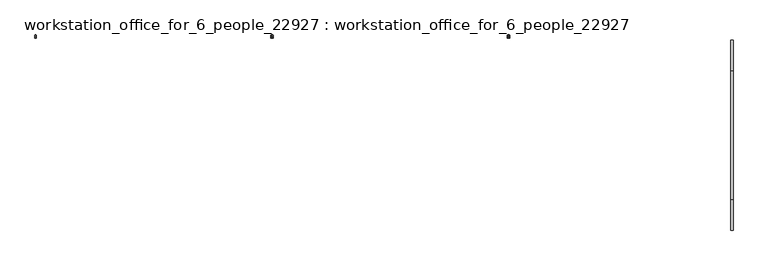
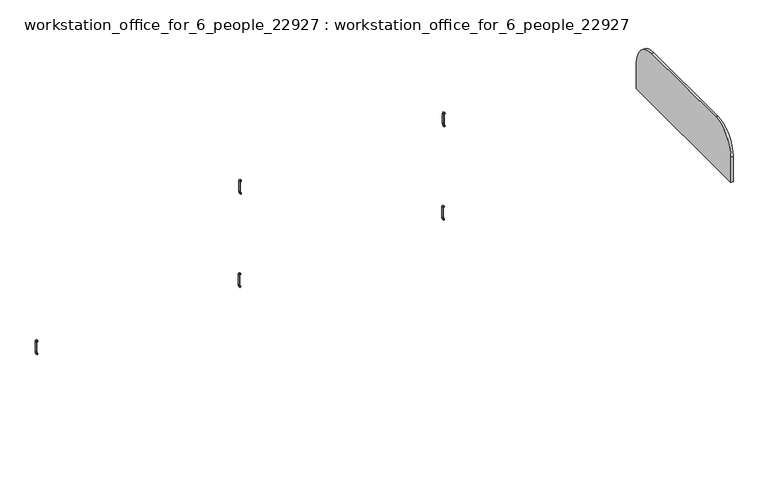
"""IFC4 building model written with IfcOpenShell, lengths in millimetres: proxy geometry, workstation_office_for_6_people_22927 : workstation_office_for_6_people_22927."""

from ifc_helpers import new_model, si_unit, point, frame, frame_2d, origin, place, context, project, spatial, polyline, circle_curve, ellipse_curve, trimmed, segment, composite_curve, outline, extrude, source, transform, mapped, element, save
from ifc_brep_helpers import plane_surface, cylinder_surface, revolved_surface, advanced_brep


def workstation_office_for_6_people_22927_workstation_office_for_d460ba9c(model_context):
    return source(origin(), model_context, "Body", "SolidModel", [
        advanced_brep(
        [(-850.0, 629.8015658, 350.0), (-850.0, 629.8015658, 360.0), (-850.0, 635.0, 360.0), (-850.0, 635.0, 350.0), (-850.0, 640.0, 345.0), (-850.0, 650.0, 345.0), (-850.0, 650.0, 265.0), (-850.0, 640.0, 265.0), (-850.0, 635.0, 260.0), (-850.0, 635.0, 250.0), (-850.0, 629.8015658, 260.0), (-850.0, 629.8015658, 250.0)],
        [
            (0, 1, circle_curve(frame((-850.0, 629.8015658, 355.0), z_axis=(0.0, -1.0, 0.0), x_axis=(0.0, 0.0, 1.0)), 5.0)),
            (1, 0, circle_curve(frame((-850.0, 629.8015658, 355.0), z_axis=(0.0, -1.0, 0.0), x_axis=(0.0, 0.0, 1.0)), 5.0)),
            (1, 2),
            (2, 3, circle_curve(frame((-850.0, 635.0, 355.0), z_axis=(0.0, -1.0, 0.0), x_axis=(0.0, 0.0, 1.0)), 5.0)),
            (3, 0),
            (3, 2, circle_curve(frame((-850.0, 635.0, 355.0), z_axis=(0.0, -1.0, 0.0), x_axis=(0.0, 0.0, 1.0)), 5.0)),
            (4, 3, circle_curve(frame((-850.0, 635.0, 345.0), z_axis=(1.0, 0.0, 0.0), x_axis=(0.0, 0.0, 1.0)), 5.0)),
            (2, 5, circle_curve(frame((-850.0, 635.0, 345.0), z_axis=(-1.0, 0.0, 0.0), x_axis=(0.0, 0.0, 1.0)), 15.0)),
            (5, 4, circle_curve(frame((-850.0, 645.0, 345.0), z_axis=(0.0, 0.0, 1.0), x_axis=(0.0, 1.0, 0.0)), 5.0)),
            (4, 5, circle_curve(frame((-850.0, 645.0, 345.0), z_axis=(0.0, 0.0, 1.0), x_axis=(0.0, 1.0, 0.0)), 5.0)),
            (5, 6),
            (6, 7, circle_curve(frame((-850.0, 645.0, 265.0), z_axis=(0.0, 0.0, 1.0), x_axis=(0.0, 1.0, 0.0)), 5.0)),
            (7, 4),
            (7, 6, circle_curve(frame((-850.0, 645.0, 265.0), z_axis=(0.0, 0.0, 1.0), x_axis=(0.0, 1.0, 0.0)), 5.0)),
            (8, 7, circle_curve(frame((-850.0, 635.0, 265.0), z_axis=(1.0, 0.0, 0.0), x_axis=(0.0, 1.0, 0.0)), 5.0)),
            (6, 9, circle_curve(frame((-850.0, 635.0, 265.0), z_axis=(-1.0, 0.0, 0.0), x_axis=(0.0, 1.0, 0.0)), 15.0)),
            (9, 8, circle_curve(frame((-850.0, 635.0, 255.0), z_axis=(0.0, 1.0, 0.0), x_axis=(0.0, 0.0, -1.0)), 5.0)),
            (8, 9, circle_curve(frame((-850.0, 635.0, 255.0), z_axis=(0.0, 1.0, 0.0), x_axis=(0.0, 0.0, -1.0)), 5.0)),
            (10, 11, circle_curve(frame((-850.0, 629.8015658, 255.0), z_axis=(0.0, -1.0, 0.0), x_axis=(0.0, 0.0, -1.0)), 5.0)),
            (11, 10, circle_curve(frame((-850.0, 629.8015658, 255.0), z_axis=(0.0, -1.0, 0.0), x_axis=(0.0, 0.0, -1.0)), 5.0)),
            (9, 11),
            (10, 8),
        ],
        [
            plane_surface(frame((0.0, 629.8015658, 355.0), z_axis=(0.0, -1.0, 0.0), x_axis=(1.0, 0.0, 0.0))),
            cylinder_surface(frame((-850.0, 629.8015658, 355.0), z_axis=(0.0, -1.0, 0.0), x_axis=(0.0, 0.0, 1.0)), 5.0),
            revolved_surface(trimmed(ellipse_curve(frame((-850.0, 635.0, 355.0), z_axis=(0.0, -1.0, 0.0), x_axis=(0.0, 0.0, 1.0)), 5.0, 5.0), [point((-850.0, 635.0, 360.0))], [point((-850.0, 635.0, 350.0))], True, "CARTESIAN"), (0.0, 635.0, 345.0), (-1.0, 0.0, 0.0)),
            revolved_surface(trimmed(ellipse_curve(frame((-850.0, 635.0, 355.0), z_axis=(0.0, -1.0, 0.0), x_axis=(0.0, 0.0, 1.0)), 5.0, 5.0), [point((-850.0, 635.0, 350.0))], [point((-850.0, 635.0, 360.0))], True, "CARTESIAN"), (0.0, 635.0, 345.0), (-1.0, 0.0, 0.0)),
            cylinder_surface(frame((-850.0, 645.0, 345.0), z_axis=(0.0, 0.0, 1.0), x_axis=(0.0, 1.0, 0.0)), 5.0),
            revolved_surface(trimmed(ellipse_curve(frame((-850.0, 645.0, 265.0), z_axis=(0.0, 0.0, 1.0), x_axis=(0.0, 1.0, 0.0)), 5.0, 5.0), [point((-850.0, 650.0, 265.0))], [point((-850.0, 640.0, 265.0))], True, "CARTESIAN"), (0.0, 635.0, 265.0), (-1.0, 0.0, 0.0)),
            revolved_surface(trimmed(ellipse_curve(frame((-850.0, 645.0, 265.0), z_axis=(0.0, 0.0, 1.0), x_axis=(0.0, 1.0, 0.0)), 5.0, 5.0), [point((-850.0, 640.0, 265.0))], [point((-850.0, 650.0, 265.0))], True, "CARTESIAN"), (0.0, 635.0, 265.0), (-1.0, 0.0, 0.0)),
            plane_surface(frame((0.0, 629.8015658, 255.0), z_axis=(0.0, -1.0, 0.0), x_axis=(1.0, 0.0, 0.0))),
            cylinder_surface(frame((-850.0, 635.0, 255.0), z_axis=(0.0, 1.0, 0.0), x_axis=(0.0, 0.0, -1.0)), 5.0),
        ],
        [
            (0, [[1, 2]]),
            (1, [[-2, 3, 4, 5]]),
            (1, [[-1, -5, 6, -3]]),
            (2, [[7, -4, 8, 9]]),
            (3, [[-8, -6, -7, 10]]),
            (4, [[-9, 11, 12, 13]]),
            (4, [[-10, -13, 14, -11]]),
            (5, [[15, -12, 16, 17]]),
            (6, [[-16, -14, -15, 18]]),
            (7, [[19, 20]]),
            (8, [[-17, 21, -19, 22]]),
            (8, [[-18, -22, -20, -21]]),
        ],
    ),
        advanced_brep(
        [(680.0, 629.8015658, 1090.0), (680.0, 629.8015658, 1100.0), (680.0, 635.0, 1100.0), (680.0, 635.0, 1090.0), (680.0, 640.0, 1085.0), (680.0, 650.0, 1085.0), (680.0, 650.0, 1005.0), (680.0, 640.0, 1005.0), (680.0, 635.0, 1000.0), (680.0, 635.0, 990.0), (680.0, 629.8015658, 1000.0), (680.0, 629.8015658, 990.0)],
        [
            (0, 1, circle_curve(frame((680.0, 629.8015658, 1095.0), z_axis=(0.0, -1.0, 0.0), x_axis=(0.0, 0.0, 1.0)), 5.0)),
            (1, 0, circle_curve(frame((680.0, 629.8015658, 1095.0), z_axis=(0.0, -1.0, 0.0), x_axis=(0.0, 0.0, 1.0)), 5.0)),
            (1, 2),
            (2, 3, circle_curve(frame((680.0, 635.0, 1095.0), z_axis=(0.0, -1.0, 0.0), x_axis=(0.0, 0.0, 1.0)), 5.0)),
            (3, 0),
            (3, 2, circle_curve(frame((680.0, 635.0, 1095.0), z_axis=(0.0, -1.0, 0.0), x_axis=(0.0, 0.0, 1.0)), 5.0)),
            (4, 3, circle_curve(frame((680.0, 635.0, 1085.0), z_axis=(1.0, 0.0, 0.0), x_axis=(0.0, 0.0, 1.0)), 5.0)),
            (2, 5, circle_curve(frame((680.0, 635.0, 1085.0), z_axis=(-1.0, 0.0, 0.0), x_axis=(0.0, 0.0, 1.0)), 15.0)),
            (5, 4, circle_curve(frame((680.0, 645.0, 1085.0), z_axis=(0.0, 0.0, 1.0), x_axis=(0.0, 1.0, 0.0)), 5.0)),
            (4, 5, circle_curve(frame((680.0, 645.0, 1085.0), z_axis=(0.0, 0.0, 1.0), x_axis=(0.0, 1.0, 0.0)), 5.0)),
            (5, 6),
            (6, 7, circle_curve(frame((680.0, 645.0, 1005.0), z_axis=(0.0, 0.0, 1.0), x_axis=(0.0, 1.0, 0.0)), 5.0)),
            (7, 4),
            (7, 6, circle_curve(frame((680.0, 645.0, 1005.0), z_axis=(0.0, 0.0, 1.0), x_axis=(0.0, 1.0, 0.0)), 5.0)),
            (8, 7, circle_curve(frame((680.0, 635.0, 1005.0), z_axis=(1.0, 0.0, 0.0), x_axis=(0.0, 1.0, 0.0)), 5.0)),
            (6, 9, circle_curve(frame((680.0, 635.0, 1005.0), z_axis=(-1.0, 0.0, 0.0), x_axis=(0.0, 1.0, 0.0)), 15.0)),
            (9, 8, circle_curve(frame((680.0, 635.0, 995.0), z_axis=(0.0, 1.0, 0.0), x_axis=(0.0, 0.0, -1.0)), 5.0)),
            (8, 9, circle_curve(frame((680.0, 635.0, 995.0), z_axis=(0.0, 1.0, 0.0), x_axis=(0.0, 0.0, -1.0)), 5.0)),
            (10, 11, circle_curve(frame((680.0, 629.8015658, 995.0), z_axis=(0.0, -1.0, 0.0), x_axis=(0.0, 0.0, -1.0)), 5.0)),
            (11, 10, circle_curve(frame((680.0, 629.8015658, 995.0), z_axis=(0.0, -1.0, 0.0), x_axis=(0.0, 0.0, -1.0)), 5.0)),
            (9, 11),
            (10, 8),
        ],
        [
            plane_surface(frame((1530.0, 629.8015658, 1095.0), z_axis=(0.0, -1.0, 0.0), x_axis=(1.0, 0.0, 0.0))),
            cylinder_surface(frame((680.0, 629.8015658, 1095.0), z_axis=(0.0, -1.0, 0.0), x_axis=(0.0, 0.0, 1.0)), 5.0),
            revolved_surface(trimmed(ellipse_curve(frame((680.0, 635.0, 1095.0), z_axis=(0.0, -1.0, 0.0), x_axis=(0.0, 0.0, 1.0)), 5.0, 5.0), [point((680.0, 635.0, 1100.0))], [point((680.0, 635.0, 1090.0))], True, "CARTESIAN"), (1530.0, 635.0, 1085.0), (-1.0, 0.0, 0.0)),
            revolved_surface(trimmed(ellipse_curve(frame((680.0, 635.0, 1095.0), z_axis=(0.0, -1.0, 0.0), x_axis=(0.0, 0.0, 1.0)), 5.0, 5.0), [point((680.0, 635.0, 1090.0))], [point((680.0, 635.0, 1100.0))], True, "CARTESIAN"), (1530.0, 635.0, 1085.0), (-1.0, 0.0, 0.0)),
            cylinder_surface(frame((680.0, 645.0, 1085.0), z_axis=(0.0, 0.0, 1.0), x_axis=(0.0, 1.0, 0.0)), 5.0),
            revolved_surface(trimmed(ellipse_curve(frame((680.0, 645.0, 1005.0), z_axis=(0.0, 0.0, 1.0), x_axis=(0.0, 1.0, 0.0)), 5.0, 5.0), [point((680.0, 650.0, 1005.0))], [point((680.0, 640.0, 1005.0))], True, "CARTESIAN"), (1530.0, 635.0, 1005.0), (-1.0, 0.0, 0.0)),
            revolved_surface(trimmed(ellipse_curve(frame((680.0, 645.0, 1005.0), z_axis=(0.0, 0.0, 1.0), x_axis=(0.0, 1.0, 0.0)), 5.0, 5.0), [point((680.0, 640.0, 1005.0))], [point((680.0, 650.0, 1005.0))], True, "CARTESIAN"), (1530.0, 635.0, 1005.0), (-1.0, 0.0, 0.0)),
            plane_surface(frame((1530.0, 629.8015658, 995.0), z_axis=(0.0, -1.0, 0.0), x_axis=(1.0, 0.0, 0.0))),
            cylinder_surface(frame((680.0, 635.0, 995.0), z_axis=(0.0, 1.0, 0.0), x_axis=(0.0, 0.0, -1.0)), 5.0),
        ],
        [
            (0, [[1, 2]]),
            (1, [[-2, 3, 4, 5]]),
            (1, [[-1, -5, 6, -3]]),
            (2, [[7, -4, 8, 9]]),
            (3, [[-8, -6, -7, 10]]),
            (4, [[-9, 11, 12, 13]]),
            (4, [[-10, -13, 14, -11]]),
            (5, [[15, -12, 16, 17]]),
            (6, [[-16, -14, -15, 18]]),
            (7, [[19, 20]]),
            (8, [[-17, 21, -19, 22]]),
            (8, [[-18, -22, -20, -21]]),
        ],
    ),
        advanced_brep(
        [(675.0, 629.8015658, 350.0), (675.0, 629.8015658, 360.0), (675.0, 635.0, 360.0), (675.0, 635.0, 350.0), (675.0, 640.0, 345.0), (675.0, 650.0, 345.0), (675.0, 650.0, 265.0), (675.0, 640.0, 265.0), (675.0, 635.0, 260.0), (675.0, 635.0, 250.0), (675.0, 629.8015658, 260.0), (675.0, 629.8015658, 250.0)],
        [
            (0, 1, circle_curve(frame((675.0, 629.8015658, 355.0), z_axis=(0.0, -1.0, 0.0), x_axis=(0.0, 0.0, 1.0)), 5.0)),
            (1, 0, circle_curve(frame((675.0, 629.8015658, 355.0), z_axis=(0.0, -1.0, 0.0), x_axis=(0.0, 0.0, 1.0)), 5.0)),
            (1, 2),
            (2, 3, circle_curve(frame((675.0, 635.0, 355.0), z_axis=(0.0, -1.0, 0.0), x_axis=(0.0, 0.0, 1.0)), 5.0)),
            (3, 0),
            (3, 2, circle_curve(frame((675.0, 635.0, 355.0), z_axis=(0.0, -1.0, 0.0), x_axis=(0.0, 0.0, 1.0)), 5.0)),
            (4, 3, circle_curve(frame((675.0, 635.0, 345.0), z_axis=(1.0, 0.0, 0.0), x_axis=(0.0, 0.0, 1.0)), 5.0)),
            (2, 5, circle_curve(frame((675.0, 635.0, 345.0), z_axis=(-1.0, 0.0, 0.0), x_axis=(0.0, 0.0, 1.0)), 15.0)),
            (5, 4, circle_curve(frame((675.0, 645.0, 345.0), z_axis=(0.0, 0.0, 1.0), x_axis=(0.0, 1.0, 0.0)), 5.0)),
            (4, 5, circle_curve(frame((675.0, 645.0, 345.0), z_axis=(0.0, 0.0, 1.0), x_axis=(0.0, 1.0, 0.0)), 5.0)),
            (5, 6),
            (6, 7, circle_curve(frame((675.0, 645.0, 265.0), z_axis=(0.0, 0.0, 1.0), x_axis=(0.0, 1.0, 0.0)), 5.0)),
            (7, 4),
            (7, 6, circle_curve(frame((675.0, 645.0, 265.0), z_axis=(0.0, 0.0, 1.0), x_axis=(0.0, 1.0, 0.0)), 5.0)),
            (8, 7, circle_curve(frame((675.0, 635.0, 265.0), z_axis=(1.0, 0.0, 0.0), x_axis=(0.0, 1.0, 0.0)), 5.0)),
            (6, 9, circle_curve(frame((675.0, 635.0, 265.0), z_axis=(-1.0, 0.0, 0.0), x_axis=(0.0, 1.0, 0.0)), 15.0)),
            (9, 8, circle_curve(frame((675.0, 635.0, 255.0), z_axis=(0.0, 1.0, 0.0), x_axis=(0.0, 0.0, -1.0)), 5.0)),
            (8, 9, circle_curve(frame((675.0, 635.0, 255.0), z_axis=(0.0, 1.0, 0.0), x_axis=(0.0, 0.0, -1.0)), 5.0)),
            (10, 11, circle_curve(frame((675.0, 629.8015658, 255.0), z_axis=(0.0, -1.0, 0.0), x_axis=(0.0, 0.0, -1.0)), 5.0)),
            (11, 10, circle_curve(frame((675.0, 629.8015658, 255.0), z_axis=(0.0, -1.0, 0.0), x_axis=(0.0, 0.0, -1.0)), 5.0)),
            (9, 11),
            (10, 8),
        ],
        [
            plane_surface(frame((675.0, 629.8015658, 355.0), z_axis=(0.0, -1.0, 0.0), x_axis=(1.0, 0.0, 0.0))),
            cylinder_surface(frame((675.0, 629.8015658, 355.0), z_axis=(0.0, -1.0, 0.0), x_axis=(0.0, 0.0, 1.0)), 5.0),
            revolved_surface(trimmed(ellipse_curve(frame((675.0, 635.0, 355.0), z_axis=(0.0, -1.0, 0.0), x_axis=(0.0, 0.0, 1.0)), 5.0, 5.0), [point((675.0, 635.0, 360.0))], [point((675.0, 635.0, 350.0))], True, "CARTESIAN"), (675.0, 635.0, 345.0), (-1.0, 0.0, 0.0)),
            revolved_surface(trimmed(ellipse_curve(frame((675.0, 635.0, 355.0), z_axis=(0.0, -1.0, 0.0), x_axis=(0.0, 0.0, 1.0)), 5.0, 5.0), [point((675.0, 635.0, 350.0))], [point((675.0, 635.0, 360.0))], True, "CARTESIAN"), (675.0, 635.0, 345.0), (-1.0, 0.0, 0.0)),
            cylinder_surface(frame((675.0, 645.0, 345.0), z_axis=(0.0, 0.0, 1.0), x_axis=(0.0, 1.0, 0.0)), 5.0),
            revolved_surface(trimmed(ellipse_curve(frame((675.0, 645.0, 265.0), z_axis=(0.0, 0.0, 1.0), x_axis=(0.0, 1.0, 0.0)), 5.0, 5.0), [point((675.0, 650.0, 265.0))], [point((675.0, 640.0, 265.0))], True, "CARTESIAN"), (675.0, 635.0, 265.0), (-1.0, 0.0, 0.0)),
            revolved_surface(trimmed(ellipse_curve(frame((675.0, 645.0, 265.0), z_axis=(0.0, 0.0, 1.0), x_axis=(0.0, 1.0, 0.0)), 5.0, 5.0), [point((675.0, 640.0, 265.0))], [point((675.0, 650.0, 265.0))], True, "CARTESIAN"), (675.0, 635.0, 265.0), (-1.0, 0.0, 0.0)),
            plane_surface(frame((675.0, 629.8015658, 255.0), z_axis=(0.0, -1.0, 0.0), x_axis=(1.0, 0.0, 0.0))),
            cylinder_surface(frame((675.0, 635.0, 255.0), z_axis=(0.0, 1.0, 0.0), x_axis=(0.0, 0.0, -1.0)), 5.0),
        ],
        [
            (0, [[1, 2]]),
            (1, [[-2, 3, 4, 5]]),
            (1, [[-1, -5, 6, -3]]),
            (2, [[7, -4, 8, 9]]),
            (3, [[-8, -6, -7, 10]]),
            (4, [[-9, 11, 12, 13]]),
            (4, [[-10, -13, 14, -11]]),
            (5, [[15, -12, 16, 17]]),
            (6, [[-16, -14, -15, 18]]),
            (7, [[19, 20]]),
            (8, [[-17, 21, -19, 22]]),
            (8, [[-18, -22, -20, -21]]),
        ],
    ),
        advanced_brep(
        [(2210.0, 629.8015658, 1090.0), (2210.0, 629.8015658, 1100.0), (2210.0, 635.0, 1100.0), (2210.0, 635.0, 1090.0), (2210.0, 640.0, 1085.0), (2210.0, 650.0, 1085.0), (2210.0, 650.0, 1005.0), (2210.0, 640.0, 1005.0), (2210.0, 635.0, 1000.0), (2210.0, 635.0, 990.0), (2210.0, 629.8015658, 1000.0), (2210.0, 629.8015658, 990.0)],
        [
            (0, 1, circle_curve(frame((2210.0, 629.8015658, 1095.0), z_axis=(0.0, -1.0, 0.0), x_axis=(0.0, 0.0, 1.0)), 5.0)),
            (1, 0, circle_curve(frame((2210.0, 629.8015658, 1095.0), z_axis=(0.0, -1.0, 0.0), x_axis=(0.0, 0.0, 1.0)), 5.0)),
            (1, 2),
            (2, 3, circle_curve(frame((2210.0, 635.0, 1095.0), z_axis=(0.0, -1.0, 0.0), x_axis=(0.0, 0.0, 1.0)), 5.0)),
            (3, 0),
            (3, 2, circle_curve(frame((2210.0, 635.0, 1095.0), z_axis=(0.0, -1.0, 0.0), x_axis=(0.0, 0.0, 1.0)), 5.0)),
            (4, 3, circle_curve(frame((2210.0, 635.0, 1085.0), z_axis=(1.0, 0.0, 0.0), x_axis=(0.0, 0.0, 1.0)), 5.0)),
            (2, 5, circle_curve(frame((2210.0, 635.0, 1085.0), z_axis=(-1.0, 0.0, 0.0), x_axis=(0.0, 0.0, 1.0)), 15.0)),
            (5, 4, circle_curve(frame((2210.0, 645.0, 1085.0), z_axis=(0.0, 0.0, 1.0), x_axis=(0.0, 1.0, 0.0)), 5.0)),
            (4, 5, circle_curve(frame((2210.0, 645.0, 1085.0), z_axis=(0.0, 0.0, 1.0), x_axis=(0.0, 1.0, 0.0)), 5.0)),
            (5, 6),
            (6, 7, circle_curve(frame((2210.0, 645.0, 1005.0), z_axis=(0.0, 0.0, 1.0), x_axis=(0.0, 1.0, 0.0)), 5.0)),
            (7, 4),
            (7, 6, circle_curve(frame((2210.0, 645.0, 1005.0), z_axis=(0.0, 0.0, 1.0), x_axis=(0.0, 1.0, 0.0)), 5.0)),
            (8, 7, circle_curve(frame((2210.0, 635.0, 1005.0), z_axis=(1.0, 0.0, 0.0), x_axis=(0.0, 1.0, 0.0)), 5.0)),
            (6, 9, circle_curve(frame((2210.0, 635.0, 1005.0), z_axis=(-1.0, 0.0, 0.0), x_axis=(0.0, 1.0, 0.0)), 15.0)),
            (9, 8, circle_curve(frame((2210.0, 635.0, 995.0), z_axis=(0.0, 1.0, 0.0), x_axis=(0.0, 0.0, -1.0)), 5.0)),
            (8, 9, circle_curve(frame((2210.0, 635.0, 995.0), z_axis=(0.0, 1.0, 0.0), x_axis=(0.0, 0.0, -1.0)), 5.0)),
            (10, 11, circle_curve(frame((2210.0, 629.8015658, 995.0), z_axis=(0.0, -1.0, 0.0), x_axis=(0.0, 0.0, -1.0)), 5.0)),
            (11, 10, circle_curve(frame((2210.0, 629.8015658, 995.0), z_axis=(0.0, -1.0, 0.0), x_axis=(0.0, 0.0, -1.0)), 5.0)),
            (9, 11),
            (10, 8),
        ],
        [
            plane_surface(frame((3060.0, 629.8015658, 1095.0), z_axis=(0.0, -1.0, 0.0), x_axis=(1.0, 0.0, 0.0))),
            cylinder_surface(frame((2210.0, 629.8015658, 1095.0), z_axis=(0.0, -1.0, 0.0), x_axis=(0.0, 0.0, 1.0)), 5.0),
            revolved_surface(trimmed(ellipse_curve(frame((2210.0, 635.0, 1095.0), z_axis=(0.0, -1.0, 0.0), x_axis=(0.0, 0.0, 1.0)), 5.0, 5.0), [point((2210.0, 635.0, 1100.0))], [point((2210.0, 635.0, 1090.0))], True, "CARTESIAN"), (3060.0, 635.0, 1085.0), (-1.0, 0.0, 0.0)),
            revolved_surface(trimmed(ellipse_curve(frame((2210.0, 635.0, 1095.0), z_axis=(0.0, -1.0, 0.0), x_axis=(0.0, 0.0, 1.0)), 5.0, 5.0), [point((2210.0, 635.0, 1090.0))], [point((2210.0, 635.0, 1100.0))], True, "CARTESIAN"), (3060.0, 635.0, 1085.0), (-1.0, 0.0, 0.0)),
            cylinder_surface(frame((2210.0, 645.0, 1085.0), z_axis=(0.0, 0.0, 1.0), x_axis=(0.0, 1.0, 0.0)), 5.0),
            revolved_surface(trimmed(ellipse_curve(frame((2210.0, 645.0, 1005.0), z_axis=(0.0, 0.0, 1.0), x_axis=(0.0, 1.0, 0.0)), 5.0, 5.0), [point((2210.0, 650.0, 1005.0))], [point((2210.0, 640.0, 1005.0))], True, "CARTESIAN"), (3060.0, 635.0, 1005.0), (-1.0, 0.0, 0.0)),
            revolved_surface(trimmed(ellipse_curve(frame((2210.0, 645.0, 1005.0), z_axis=(0.0, 0.0, 1.0), x_axis=(0.0, 1.0, 0.0)), 5.0, 5.0), [point((2210.0, 640.0, 1005.0))], [point((2210.0, 650.0, 1005.0))], True, "CARTESIAN"), (3060.0, 635.0, 1005.0), (-1.0, 0.0, 0.0)),
            plane_surface(frame((3060.0, 629.8015658, 995.0), z_axis=(0.0, -1.0, 0.0), x_axis=(1.0, 0.0, 0.0))),
            cylinder_surface(frame((2210.0, 635.0, 995.0), z_axis=(0.0, 1.0, 0.0), x_axis=(0.0, 0.0, -1.0)), 5.0),
        ],
        [
            (0, [[1, 2]]),
            (1, [[-2, 3, 4, 5]]),
            (1, [[-1, -5, 6, -3]]),
            (2, [[7, -4, 8, 9]]),
            (3, [[-8, -6, -7, 10]]),
            (4, [[-9, 11, 12, 13]]),
            (4, [[-10, -13, 14, -11]]),
            (5, [[15, -12, 16, 17]]),
            (6, [[-16, -14, -15, 18]]),
            (7, [[19, 20]]),
            (8, [[-17, 21, -19, 22]]),
            (8, [[-18, -22, -20, -21]]),
        ],
    ),
        advanced_brep(
        [(2205.0, 629.8015658, 350.0), (2205.0, 629.8015658, 360.0), (2205.0, 635.0, 360.0), (2205.0, 635.0, 350.0), (2205.0, 640.0, 345.0), (2205.0, 650.0, 345.0), (2205.0, 650.0, 265.0), (2205.0, 640.0, 265.0), (2205.0, 635.0, 260.0), (2205.0, 635.0, 250.0), (2205.0, 629.8015658, 260.0), (2205.0, 629.8015658, 250.0)],
        [
            (0, 1, circle_curve(frame((2205.0, 629.8015658, 355.0), z_axis=(0.0, -1.0, 0.0), x_axis=(0.0, 0.0, 1.0)), 5.0)),
            (1, 0, circle_curve(frame((2205.0, 629.8015658, 355.0), z_axis=(0.0, -1.0, 0.0), x_axis=(0.0, 0.0, 1.0)), 5.0)),
            (1, 2),
            (2, 3, circle_curve(frame((2205.0, 635.0, 355.0), z_axis=(0.0, -1.0, 0.0), x_axis=(0.0, 0.0, 1.0)), 5.0)),
            (3, 0),
            (3, 2, circle_curve(frame((2205.0, 635.0, 355.0), z_axis=(0.0, -1.0, 0.0), x_axis=(0.0, 0.0, 1.0)), 5.0)),
            (4, 3, circle_curve(frame((2205.0, 635.0, 345.0), z_axis=(1.0, 0.0, 0.0), x_axis=(0.0, 0.0, 1.0)), 5.0)),
            (2, 5, circle_curve(frame((2205.0, 635.0, 345.0), z_axis=(-1.0, 0.0, 0.0), x_axis=(0.0, 0.0, 1.0)), 15.0)),
            (5, 4, circle_curve(frame((2205.0, 645.0, 345.0), z_axis=(0.0, 0.0, 1.0), x_axis=(0.0, 1.0, 0.0)), 5.0)),
            (4, 5, circle_curve(frame((2205.0, 645.0, 345.0), z_axis=(0.0, 0.0, 1.0), x_axis=(0.0, 1.0, 0.0)), 5.0)),
            (5, 6),
            (6, 7, circle_curve(frame((2205.0, 645.0, 265.0), z_axis=(0.0, 0.0, 1.0), x_axis=(0.0, 1.0, 0.0)), 5.0)),
            (7, 4),
            (7, 6, circle_curve(frame((2205.0, 645.0, 265.0), z_axis=(0.0, 0.0, 1.0), x_axis=(0.0, 1.0, 0.0)), 5.0)),
            (8, 7, circle_curve(frame((2205.0, 635.0, 265.0), z_axis=(1.0, 0.0, 0.0), x_axis=(0.0, 1.0, 0.0)), 5.0)),
            (6, 9, circle_curve(frame((2205.0, 635.0, 265.0), z_axis=(-1.0, 0.0, 0.0), x_axis=(0.0, 1.0, 0.0)), 15.0)),
            (9, 8, circle_curve(frame((2205.0, 635.0, 255.0), z_axis=(0.0, 1.0, 0.0), x_axis=(0.0, 0.0, -1.0)), 5.0)),
            (8, 9, circle_curve(frame((2205.0, 635.0, 255.0), z_axis=(0.0, 1.0, 0.0), x_axis=(0.0, 0.0, -1.0)), 5.0)),
            (10, 11, circle_curve(frame((2205.0, 629.8015658, 255.0), z_axis=(0.0, -1.0, 0.0), x_axis=(0.0, 0.0, -1.0)), 5.0)),
            (11, 10, circle_curve(frame((2205.0, 629.8015658, 255.0), z_axis=(0.0, -1.0, 0.0), x_axis=(0.0, 0.0, -1.0)), 5.0)),
            (9, 11),
            (10, 8),
        ],
        [
            plane_surface(frame((2205.0, 629.8015658, 355.0), z_axis=(0.0, -1.0, 0.0), x_axis=(1.0, 0.0, 0.0))),
            cylinder_surface(frame((2205.0, 629.8015658, 355.0), z_axis=(0.0, -1.0, 0.0), x_axis=(0.0, 0.0, 1.0)), 5.0),
            revolved_surface(trimmed(ellipse_curve(frame((2205.0, 635.0, 355.0), z_axis=(0.0, -1.0, 0.0), x_axis=(0.0, 0.0, 1.0)), 5.0, 5.0), [point((2205.0, 635.0, 360.0))], [point((2205.0, 635.0, 350.0))], True, "CARTESIAN"), (2205.0, 635.0, 345.0), (-1.0, 0.0, 0.0)),
            revolved_surface(trimmed(ellipse_curve(frame((2205.0, 635.0, 355.0), z_axis=(0.0, -1.0, 0.0), x_axis=(0.0, 0.0, 1.0)), 5.0, 5.0), [point((2205.0, 635.0, 350.0))], [point((2205.0, 635.0, 360.0))], True, "CARTESIAN"), (2205.0, 635.0, 345.0), (-1.0, 0.0, 0.0)),
            cylinder_surface(frame((2205.0, 645.0, 345.0), z_axis=(0.0, 0.0, 1.0), x_axis=(0.0, 1.0, 0.0)), 5.0),
            revolved_surface(trimmed(ellipse_curve(frame((2205.0, 645.0, 265.0), z_axis=(0.0, 0.0, 1.0), x_axis=(0.0, 1.0, 0.0)), 5.0, 5.0), [point((2205.0, 650.0, 265.0))], [point((2205.0, 640.0, 265.0))], True, "CARTESIAN"), (2205.0, 635.0, 265.0), (-1.0, 0.0, 0.0)),
            revolved_surface(trimmed(ellipse_curve(frame((2205.0, 645.0, 265.0), z_axis=(0.0, 0.0, 1.0), x_axis=(0.0, 1.0, 0.0)), 5.0, 5.0), [point((2205.0, 640.0, 265.0))], [point((2205.0, 650.0, 265.0))], True, "CARTESIAN"), (2205.0, 635.0, 265.0), (-1.0, 0.0, 0.0)),
            plane_surface(frame((2205.0, 629.8015658, 255.0), z_axis=(0.0, -1.0, 0.0), x_axis=(1.0, 0.0, 0.0))),
            cylinder_surface(frame((2205.0, 635.0, 255.0), z_axis=(0.0, 1.0, 0.0), x_axis=(0.0, 0.0, -1.0)), 5.0),
        ],
        [
            (0, [[1, 2]]),
            (1, [[-2, 3, 4, 5]]),
            (1, [[-1, -5, 6, -3]]),
            (2, [[7, -4, 8, 9]]),
            (3, [[-8, -6, -7, 10]]),
            (4, [[-9, 11, 12, 13]]),
            (4, [[-10, -13, 14, -11]]),
            (5, [[15, -12, 16, 17]]),
            (6, [[-16, -14, -15, 18]]),
            (7, [[19, 20]]),
            (8, [[-17, 21, -19, 22]]),
            (8, [[-18, -22, -20, -21]]),
        ],
    ),
        extrude(outline(composite_curve([segment(trimmed(circle_curve(frame_2d((415.0, 1000.0)), 200.0), [point((415.0, 1200.0))], [point((615.0, 1000.0))], False, "CARTESIAN"), True, "CONTINUOUS"), segment(polyline([(615.0, 1000.0), (615.0, 800.0), (-615.0, 800.0), (-615.0, 1000.0)]), True, "CONTINUOUS"), segment(trimmed(circle_curve(frame_2d((-415.0, 1000.0)), 200.0), [point((-615.0, 1000.0))], [point((-415.0, 1200.0))], False, "CARTESIAN"), True, "CONTINUOUS"), segment(polyline([(-415.0, 1200.0), (415.0, 1200.0)]), True, "CONTINUOUS")], self_intersect=False)), frame((3644.2536992, 0.0, 0.0), z_axis=(1.0, 0.0, 0.0), x_axis=(0.0, 1.0, 0.0)), (0.0, 0.0, 1.0), 15.7463008),
    ])


if __name__ == "__main__":
    model = new_model("IFC4")
    model_context = context("Model", 3, world=origin())
    ifc_project = project(units=[si_unit("LENGTHUNIT", "METRE", prefix="MILLI")], contexts=[model_context])
    site = spatial("IfcSite", under=ifc_project)
    building = spatial("IfcBuilding", under=site)
    placement = place(None, origin())
    workstation_office_for_6_people_22927_workstation_office_for_shape = workstation_office_for_6_people_22927_workstation_office_for_d460ba9c(model_context)
    element("IfcBuildingElementProxy", 1, Name="workstation_office_for_6_people_22927 : workstation_office_for_6_people_22927", ObjectType="workstation_office_for_6_people_22927 : workstation_office_for_6_people_22927", at=placement, inside=building, context=model_context, shape_type="MappedRepresentation", body=[
        mapped(workstation_office_for_6_people_22927_workstation_office_for_shape, transform((0.0, 0.0, 0.0), x_axis=(1.0, 0.0, 0.0), y_axis=(0.0, 1.0, 0.0), z_axis=(0.0, 0.0, 1.0))),
    ])
    save(model, "model.ifc")

# Revit data of these elements
# Type "workstation_office_for_6_people_22927 : workstation_office_for_6_people_22927"
#   Default Elevation = 0
# Element 1 (IfcBuildingElementProxy, "workstation_office_for_6_people_22927 : workstation_office_for_6_people_22927")
#   Materials on its faces: "green", "sahara", "white"
# Materials
#   "green": class "Generic", colour RGB 0 255 127, transparency 0, Cost = 0
#   "sahara": class "Generic", colour RGB 252 208 143, transparency 0, Cost = 0
#   "white": class "Generic", colour RGB 219 219 219, transparency 0, Cost = 0
